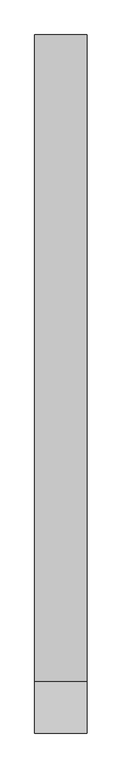
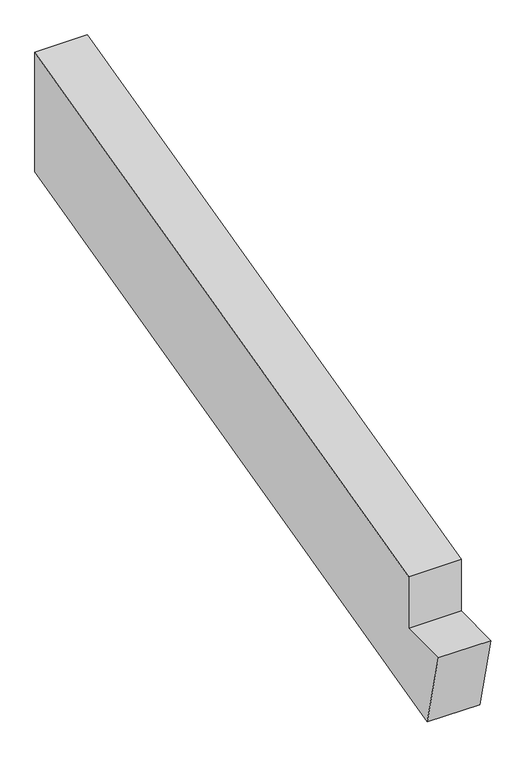
"""IFC4 building model written with IfcOpenShell, lengths in millimetres: proxy geometry, Framing025 33492 : Framing025 33492."""

from ifc_helpers import new_model, si_unit, frame, origin, place, context, project, spatial, polyline, outline, extrude, source, transform, mapped, element, save


def generic_models_fdaa2fb1(model_context):
    return source(origin(), model_context, "Body", "SweptSolid", [
        extrude(outline(polyline([(-5374.9745897, 42642.0307603), (-5224.4076049, 42642.0307603), (-5224.4076049, 42800.8143799), (-3344.6566162, 43270.717426), (-3344.6566162, 42903.8818003), (-5318.455674, 42411.3663805), (-5374.9745897, 42642.0307603)])), frame((12534.9, 0.0, 0.0), z_axis=(1.0, 0.0, 0.0), x_axis=(0.0, 1.0, 0.0)), (0.0, 0.0, 1.0), 152.4),
    ])


if __name__ == "__main__":
    model = new_model("IFC4")
    model_context = context("Model", 3, world=origin())
    ifc_project = project(units=[si_unit("LENGTHUNIT", "METRE", prefix="MILLI")], contexts=[model_context])
    site = spatial("IfcSite", under=ifc_project)
    building = spatial("IfcBuilding", under=site)
    placement = place(None, origin())
    generic_models_shape = generic_models_fdaa2fb1(model_context)
    element("IfcBuildingElementProxy", 1, Name="Framing025 33492 : Framing025 33492", ObjectType="Framing025 33492 : Framing025 33492", at=placement, inside=building, context=model_context, shape_type="MappedRepresentation", body=[
        mapped(generic_models_shape, transform((0.0, 0.0, 0.0), x_axis=(1.0, 0.0, 0.0), y_axis=(0.0, 1.0, 0.0), z_axis=(0.0, 0.0, 1.0))),
    ])
    save(model, "model.ifc")

# Revit data of these elements
# Type "Framing025 33492 : Framing025 33492"
#   NameOverride = "Framing025"
# Element 1 (IfcBuildingElementProxy, "Framing025 33492 : Framing025 33492")
#   Materials on its faces: "WOOD FRAMING (SEE STRUCT DWGS)"
# Materials
#   "WOOD FRAMING (SEE STRUCT DWGS)": class "Unassigned", colour RGB 224 188 168, transparency 0, Cost = 0
